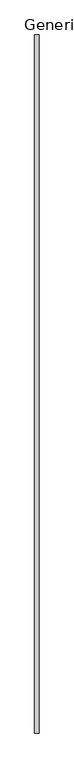
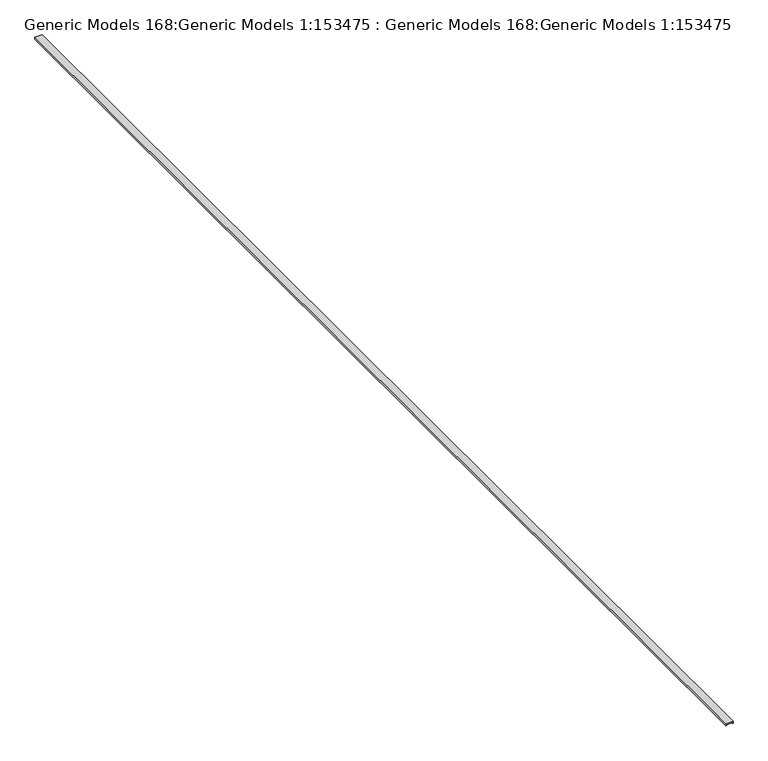
"""IFC4 building model written with IfcOpenShell, lengths in millimetres: proxy geometry, Generic Models 168:Generic Models 1:153475 : Generic Models 168:Generic Models 1:153475."""

import ifcopenshell
import ifcopenshell.guid

model = None  # the IFC model being written
_history = None  # IfcOwnerHistory: only IFC2X3 demands one
_inside = {}  # id of a spatial element -> (the spatial element, [elements in it])
_under = {}  # id of a project, library or spatial element -> (it, [spatial elements below it])
_declared = {}  # id of a project -> (the project, [libraries it declares])
_typed = {}  # id of a type object -> (the type object, [elements of that type])
_made_of = {}  # id of a material, layer set ... -> (it, [elements and type objects made of it])


def new_model(schema):
    """Start an empty IFC model of exactly this schema.

    Asked for "IFC4X3", IfcOpenShell would pick the latest addendum, in which some entities
    have other attributes; the version numbers below select the first issue.
    IFC2X3 requires an IfcOwnerHistory on every rooted entity: one is made here for all.
    """
    global model, _history
    if schema == "IFC4X3":
        model = ifcopenshell.file(schema_version=(4, 3, 0, 0))
    else:
        model = ifcopenshell.file(schema=schema)
    _inside.clear()
    _under.clear()
    _declared.clear()
    _typed.clear()
    _made_of.clear()
    _history = None
    if model.schema == "IFC2X3":
        org = make("IfcOrganization", Name="unknown")
        user = make(
            "IfcPersonAndOrganization",
            ThePerson=make("IfcPerson", FamilyName="unknown"),
            TheOrganization=org,
        )
        app = make(
            "IfcApplication",
            ApplicationDeveloper=org,
            Version="unknown",
            ApplicationFullName="unknown",
            ApplicationIdentifier="unknown",
        )
        _history = make(
            "IfcOwnerHistory",
            OwningUser=user,
            OwningApplication=app,
            ChangeAction="ADDED",
            CreationDate=0,
        )
    return model


def make(cls, **values):
    """One entity of the class cls with the attributes given. An attribute that is None is left unset."""
    return model.create_entity(
        cls, **{name: value for name, value in values.items() if value is not None}
    )


def rooted(cls, **values):
    """An entity with a GlobalId (a new one), such as an element, a storey or a relation."""
    return make(cls, GlobalId=ifcopenshell.guid.new(), OwnerHistory=_history, **values)


def si_unit(unit_type, name, prefix=None):
    """IfcSIUnit, for example si_unit("LENGTHUNIT", "METRE", prefix="MILLI")."""
    return make("IfcSIUnit", UnitType=unit_type, Prefix=prefix, Name=name)


def assignment(units):
    """IfcUnitAssignment: the units of a project."""
    return None if units is None else make("IfcUnitAssignment", Units=units)


def point(xyz):
    """IfcCartesianPoint."""
    return None if xyz is None else make("IfcCartesianPoint", Coordinates=xyz)


def direction(xyz):
    """IfcDirection."""
    return None if xyz is None else make("IfcDirection", DirectionRatios=xyz)


def frame(location, z_axis=None, x_axis=None):
    """IfcAxis2Placement3D, a coordinate frame: its origin and axes. An axis left out is left unset."""
    return make(
        "IfcAxis2Placement3D",
        Location=point(location),
        Axis=direction(z_axis),
        RefDirection=direction(x_axis),
    )


def origin():
    """The frame at (0, 0, 0) with its axes left unset."""
    return frame((0.0, 0.0, 0.0))


def place(relative_to, where):
    """IfcLocalPlacement: puts the frame where relative to a parent placement (None: the world)."""
    return make(
        "IfcLocalPlacement", PlacementRelTo=relative_to, RelativePlacement=where
    )


def context(
    kind, dimensions, precision=None, world=None, true_north=None, identifier=None
):
    """IfcGeometricRepresentationContext, for example the 3D "Model" context."""
    return make(
        "IfcGeometricRepresentationContext",
        ContextIdentifier=identifier,
        ContextType=kind,
        CoordinateSpaceDimension=dimensions,
        Precision=precision,
        WorldCoordinateSystem=world,
        TrueNorth=true_north,
    )


def project(units=None, contexts=None):
    """IfcProject with its units and contexts."""
    return rooted(
        "IfcProject",
        Name="project",
        RepresentationContexts=contexts,
        UnitsInContext=assignment(units),
    )


def spatial(cls, under=None, at=None, **own):
    """A site, building, storey or space (cls), placed at a placement, below another one or the project."""
    s = rooted(cls, ObjectPlacement=at, **own)
    if under is not None:
        _under.setdefault(under.id(), (under, []))[1].append(s)
    return s


def polyline(points):
    """IfcPolyline through the points."""
    return make("IfcPolyline", Points=[point(p) for p in points])


def outline(outer, holes=None, kind="AREA"):
    """IfcArbitraryClosedProfileDef: a profile drawn as a closed curve; with holes, ...WithVoids."""
    if holes is None:
        return make("IfcArbitraryClosedProfileDef", ProfileType=kind, OuterCurve=outer)
    return make(
        "IfcArbitraryProfileDefWithVoids",
        ProfileType=kind,
        OuterCurve=outer,
        InnerCurves=holes,
    )


def extrude(swept, where, along, depth):
    """IfcExtrudedAreaSolid: the profile swept, set in the frame where, extruded along a direction by depth."""
    return make(
        "IfcExtrudedAreaSolid",
        SweptArea=swept,
        Position=where,
        ExtrudedDirection=direction(along),
        Depth=depth,
    )


def shape(context_of_items, identifier, shape_type, items):
    """IfcShapeRepresentation: the items that make up one representation, for example the "Body"."""
    return make(
        "IfcShapeRepresentation",
        ContextOfItems=context_of_items,
        RepresentationIdentifier=identifier,
        RepresentationType=shape_type,
        Items=items,
    )


def source(mapping_origin, context_of_items, identifier, shape_type, items):
    """IfcRepresentationMap: a shape defined once, which mapped items show again and again."""
    return make(
        "IfcRepresentationMap",
        MappingOrigin=mapping_origin,
        MappedRepresentation=shape(context_of_items, identifier, shape_type, items),
    )


def transform(
    local_origin,
    x_axis=None,
    y_axis=None,
    z_axis=None,
    scale=None,
    scale2=None,
    scale3=None,
    uniform=True,
):
    """IfcCartesianTransformationOperator3D, or its non-uniform kind. x_axis, y_axis, z_axis: its Axis1, 2, 3."""
    if uniform:
        return make(
            "IfcCartesianTransformationOperator3D",
            Axis1=direction(x_axis),
            Axis2=direction(y_axis),
            LocalOrigin=point(local_origin),
            Scale=scale,
            Axis3=direction(z_axis),
        )
    return make(
        "IfcCartesianTransformationOperator3DnonUniform",
        Axis1=direction(x_axis),
        Axis2=direction(y_axis),
        LocalOrigin=point(local_origin),
        Scale=scale,
        Axis3=direction(z_axis),
        Scale2=scale2,
        Scale3=scale3,
    )


def mapped(mapping_source, mapping_target):
    """IfcMappedItem: shows the shape of a source again, moved by a transform."""
    return make(
        "IfcMappedItem", MappingSource=mapping_source, MappingTarget=mapping_target
    )


def made_of(thing, what):
    """Note that an element or type object is made of a material, layer set ...; save() writes the relation."""
    if what is not None:
        _made_of.setdefault(what.id(), (what, []))[1].append(thing)
    return thing


def element(
    cls,
    number,
    at=None,
    inside=None,
    cuts=None,
    type_object=None,
    material=None,
    context=None,
    identifier="Body",
    shape_type=None,
    held_by="IfcProductDefinitionShape",
    body=None,
    shapes=None,
    **own,
):
    """One element of the class cls, such as IfcWall. Its Tag is "e" and its number.

    at: its placement. inside: the storey or other place that contains it. cuts: it is an
    opening in that element (IfcRelVoidsElement). A single representation is given by context,
    identifier, shape_type and body (its items); several are given by shapes. held_by: the class
    of the entity that holds the representations. save() writes the other relations.
    """
    e = rooted(cls, Tag="e%d" % number, ObjectPlacement=at, **own)
    if body is not None:
        shapes = [shape(context, identifier, shape_type, body)]
    if shapes is not None:
        e.Representation = make(held_by, Representations=shapes)
    if inside is not None:
        _inside.setdefault(inside.id(), (inside, []))[1].append(e)
    if cuts is not None:
        rooted(
            "IfcRelVoidsElement", RelatingBuildingElement=cuts, RelatedOpeningElement=e
        )
    if type_object is not None:
        _typed.setdefault(type_object.id(), (type_object, []))[1].append(e)
    return made_of(e, material)


def aggregate(whole, parts):
    """IfcRelAggregates: a whole, such as a stair, and the parts it consists of."""
    return rooted("IfcRelAggregates", RelatingObject=whole, RelatedObjects=parts)


def save(model, path):
    """Write the relations noted so far, then the file.

    IfcRelAggregates (storeys below a building ...), IfcRelContainedInSpatialStructure (elements
    in a storey), IfcRelDefinesByType, IfcRelAssociatesMaterial and IfcRelDeclares: one each for
    every whole, place, type object, material and project.
    """
    for whole, parts in _under.values():
        aggregate(whole, parts)
    for where, things in _inside.values():
        rooted(
            "IfcRelContainedInSpatialStructure",
            RelatedElements=things,
            RelatingStructure=where,
        )
    for kind, things in _typed.values():
        rooted("IfcRelDefinesByType", RelatedObjects=things, RelatingType=kind)
    for what, things in _made_of.values():
        rooted("IfcRelAssociatesMaterial", RelatedObjects=things, RelatingMaterial=what)
    for by, libraries in _declared.values():
        rooted("IfcRelDeclares", RelatingContext=by, RelatedDefinitions=libraries)
    model.write(path)


def generic_models_168_generic_models_1_153475_generic_models_f00efbe0(model_context):
    return source(origin(), model_context, "Body", "SweptSolid", [
        extrude(outline(polyline([(4536.638216, -8263.059287), (4555.688216, -8263.059287), (4555.688216, -8329.734287), (4536.638216, -8329.734287), (4536.638216, -8321.796787), (4542.988216, -8321.796787), (4542.988216, -8270.996787), (4536.638216, -8270.996787), (4536.638216, -8263.059287)])), frame((0.0, -1809.1200567, 0.0), z_axis=(0.0, 1.0, 0.0), x_axis=(0.0, 0.0, 1.0)), (0.0, 0.0, 1.0), 10820.4),
    ])


if __name__ == "__main__":
    model = new_model("IFC4")
    model_context = context("Model", 3, world=origin())
    ifc_project = project(units=[si_unit("LENGTHUNIT", "METRE", prefix="MILLI")], contexts=[model_context])
    site = spatial("IfcSite", under=ifc_project)
    building = spatial("IfcBuilding", under=site)
    placement = place(None, origin())
    generic_models_168_generic_models_1_153475_generic_models_shape = generic_models_168_generic_models_1_153475_generic_models_f00efbe0(model_context)
    element("IfcBuildingElementProxy", 1, Name="Generic Models 168:Generic Models 1:153475 : Generic Models 168:Generic Models 1:153475", ObjectType="Generic Models 168:Generic Models 1:153475 : Generic Models 168:Generic Models 1:153475", at=placement, inside=building, context=model_context, shape_type="MappedRepresentation", body=[
        mapped(generic_models_168_generic_models_1_153475_generic_models_shape, transform((0.0, 0.0, 0.0), x_axis=(1.0, 0.0, 0.0), y_axis=(0.0, 1.0, 0.0), z_axis=(0.0, 0.0, 1.0))),
    ])
    save(model, "model.ifc")

# Revit data of these elements
# Type "Generic Models 168:Generic Models 1:153475 : Generic Models 168:Generic Models 1:153475"
#   NameOverride = "Generic Models 168:Generic Models 1:153475"
#   ObjectTypeOverride = "Generic Models 168:Generic Models 1"
#   Reference = "Generic Models 1"
#   Category = "Generic Models"
#   Tag = "153475"
# Element 1 (IfcBuildingElementProxy, "Generic Models 168:Generic Models 1:153475 : Generic Models 168:Generic Models 1:153475")
#   Materials on its faces: "_2 5/8\" X 3/4\" WOOD TOP RAIL / HAND RAIL, EASE EDGES W/ .01 RADIUS 13878"
# Materials
#   "_2 5/8\" X 3/4\" WOOD TOP RAIL / HAND RAIL, EASE EDGES W/ .01 RADIUS 13878": class "Unassigned", colour RGB 177 130 114, transparency 0
